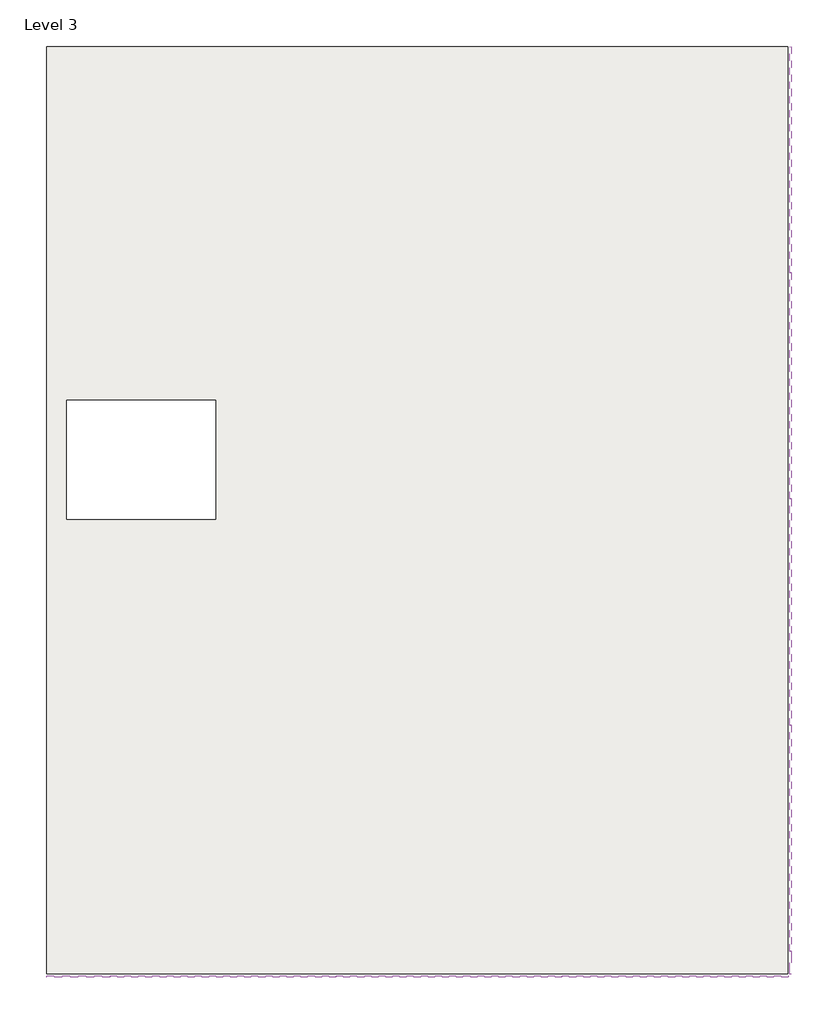
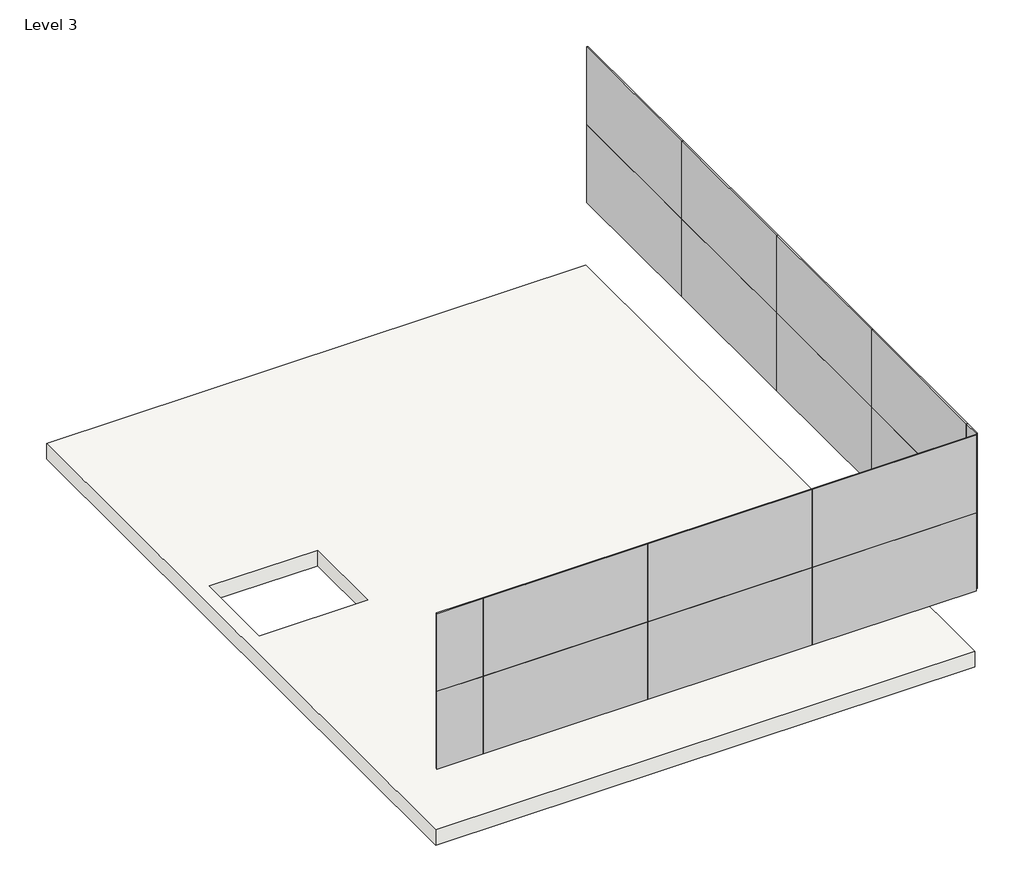
# One storey: 18 plates, 1 slab.
"""IFC4 building model written with IfcOpenShell, lengths in millimetres."""

import ifcopenshell
import ifcopenshell.guid

model = None  # the IFC model being written
_history = None  # IfcOwnerHistory: only IFC2X3 demands one
_inside = {}  # id of a spatial element -> (the spatial element, [elements in it])
_under = {}  # id of a project, library or spatial element -> (it, [spatial elements below it])
_declared = {}  # id of a project -> (the project, [libraries it declares])
_typed = {}  # id of a type object -> (the type object, [elements of that type])
_made_of = {}  # id of a material, layer set ... -> (it, [elements and type objects made of it])


def new_model(schema):
    """Start an empty IFC model of exactly this schema.

    Asked for "IFC4X3", IfcOpenShell would pick the latest addendum, in which some entities
    have other attributes; the version numbers below select the first issue.
    IFC2X3 requires an IfcOwnerHistory on every rooted entity: one is made here for all.
    """
    global model, _history
    if schema == "IFC4X3":
        model = ifcopenshell.file(schema_version=(4, 3, 0, 0))
    else:
        model = ifcopenshell.file(schema=schema)
    _inside.clear()
    _under.clear()
    _declared.clear()
    _typed.clear()
    _made_of.clear()
    _history = None
    if model.schema == "IFC2X3":
        org = make("IfcOrganization", Name="unknown")
        user = make(
            "IfcPersonAndOrganization",
            ThePerson=make("IfcPerson", FamilyName="unknown"),
            TheOrganization=org,
        )
        app = make(
            "IfcApplication",
            ApplicationDeveloper=org,
            Version="unknown",
            ApplicationFullName="unknown",
            ApplicationIdentifier="unknown",
        )
        _history = make(
            "IfcOwnerHistory",
            OwningUser=user,
            OwningApplication=app,
            ChangeAction="ADDED",
            CreationDate=0,
        )
    return model


def make(cls, **values):
    """One entity of the class cls with the attributes given. An attribute that is None is left unset."""
    return model.create_entity(
        cls, **{name: value for name, value in values.items() if value is not None}
    )


def rooted(cls, **values):
    """An entity with a GlobalId (a new one), such as an element, a storey or a relation."""
    return make(cls, GlobalId=ifcopenshell.guid.new(), OwnerHistory=_history, **values)


def si_unit(unit_type, name, prefix=None):
    """IfcSIUnit, for example si_unit("LENGTHUNIT", "METRE", prefix="MILLI")."""
    return make("IfcSIUnit", UnitType=unit_type, Prefix=prefix, Name=name)


def assignment(units):
    """IfcUnitAssignment: the units of a project."""
    return None if units is None else make("IfcUnitAssignment", Units=units)


def point(xyz):
    """IfcCartesianPoint."""
    return None if xyz is None else make("IfcCartesianPoint", Coordinates=xyz)


def direction(xyz):
    """IfcDirection."""
    return None if xyz is None else make("IfcDirection", DirectionRatios=xyz)


def frame(location, z_axis=None, x_axis=None):
    """IfcAxis2Placement3D, a coordinate frame: its origin and axes. An axis left out is left unset."""
    return make(
        "IfcAxis2Placement3D",
        Location=point(location),
        Axis=direction(z_axis),
        RefDirection=direction(x_axis),
    )


def origin():
    """The frame at (0, 0, 0) with its axes left unset."""
    return frame((0.0, 0.0, 0.0))


def origin_with_axes():
    """The frame at (0, 0, 0) with the z axis (0, 0, 1) and the x axis (1, 0, 0) written out."""
    return frame((0.0, 0.0, 0.0), z_axis=(0.0, 0.0, 1.0), x_axis=(1.0, 0.0, 0.0))


def place(relative_to, where):
    """IfcLocalPlacement: puts the frame where relative to a parent placement (None: the world)."""
    return make(
        "IfcLocalPlacement", PlacementRelTo=relative_to, RelativePlacement=where
    )


def context(
    kind, dimensions, precision=None, world=None, true_north=None, identifier=None
):
    """IfcGeometricRepresentationContext, for example the 3D "Model" context."""
    return make(
        "IfcGeometricRepresentationContext",
        ContextIdentifier=identifier,
        ContextType=kind,
        CoordinateSpaceDimension=dimensions,
        Precision=precision,
        WorldCoordinateSystem=world,
        TrueNorth=true_north,
    )


def project(units=None, contexts=None):
    """IfcProject with its units and contexts."""
    return rooted(
        "IfcProject",
        Name="project",
        RepresentationContexts=contexts,
        UnitsInContext=assignment(units),
    )


def spatial(cls, under=None, at=None, **own):
    """A site, building, storey or space (cls), placed at a placement, below another one or the project."""
    s = rooted(cls, ObjectPlacement=at, **own)
    if under is not None:
        _under.setdefault(under.id(), (under, []))[1].append(s)
    return s


def polyline(points):
    """IfcPolyline through the points."""
    return make("IfcPolyline", Points=[point(p) for p in points])


def outline(outer, holes=None, kind="AREA"):
    """IfcArbitraryClosedProfileDef: a profile drawn as a closed curve; with holes, ...WithVoids."""
    if holes is None:
        return make("IfcArbitraryClosedProfileDef", ProfileType=kind, OuterCurve=outer)
    return make(
        "IfcArbitraryProfileDefWithVoids",
        ProfileType=kind,
        OuterCurve=outer,
        InnerCurves=holes,
    )


def extrude(swept, where, along, depth):
    """IfcExtrudedAreaSolid: the profile swept, set in the frame where, extruded along a direction by depth."""
    return make(
        "IfcExtrudedAreaSolid",
        SweptArea=swept,
        Position=where,
        ExtrudedDirection=direction(along),
        Depth=depth,
    )


def shape(context_of_items, identifier, shape_type, items):
    """IfcShapeRepresentation: the items that make up one representation, for example the "Body"."""
    return make(
        "IfcShapeRepresentation",
        ContextOfItems=context_of_items,
        RepresentationIdentifier=identifier,
        RepresentationType=shape_type,
        Items=items,
    )


def source(mapping_origin, context_of_items, identifier, shape_type, items):
    """IfcRepresentationMap: a shape defined once, which mapped items show again and again."""
    return make(
        "IfcRepresentationMap",
        MappingOrigin=mapping_origin,
        MappedRepresentation=shape(context_of_items, identifier, shape_type, items),
    )


def transform(
    local_origin,
    x_axis=None,
    y_axis=None,
    z_axis=None,
    scale=None,
    scale2=None,
    scale3=None,
    uniform=True,
):
    """IfcCartesianTransformationOperator3D, or its non-uniform kind. x_axis, y_axis, z_axis: its Axis1, 2, 3."""
    if uniform:
        return make(
            "IfcCartesianTransformationOperator3D",
            Axis1=direction(x_axis),
            Axis2=direction(y_axis),
            LocalOrigin=point(local_origin),
            Scale=scale,
            Axis3=direction(z_axis),
        )
    return make(
        "IfcCartesianTransformationOperator3DnonUniform",
        Axis1=direction(x_axis),
        Axis2=direction(y_axis),
        LocalOrigin=point(local_origin),
        Scale=scale,
        Axis3=direction(z_axis),
        Scale2=scale2,
        Scale3=scale3,
    )


def mapped(mapping_source, mapping_target):
    """IfcMappedItem: shows the shape of a source again, moved by a transform."""
    return make(
        "IfcMappedItem", MappingSource=mapping_source, MappingTarget=mapping_target
    )


def made_of(thing, what):
    """Note that an element or type object is made of a material, layer set ...; save() writes the relation."""
    if what is not None:
        _made_of.setdefault(what.id(), (what, []))[1].append(thing)
    return thing


def element(
    cls,
    number,
    at=None,
    inside=None,
    cuts=None,
    type_object=None,
    material=None,
    context=None,
    identifier="Body",
    shape_type=None,
    held_by="IfcProductDefinitionShape",
    body=None,
    shapes=None,
    **own,
):
    """One element of the class cls, such as IfcWall. Its Tag is "e" and its number.

    at: its placement. inside: the storey or other place that contains it. cuts: it is an
    opening in that element (IfcRelVoidsElement). A single representation is given by context,
    identifier, shape_type and body (its items); several are given by shapes. held_by: the class
    of the entity that holds the representations. save() writes the other relations.
    """
    e = rooted(cls, Tag="e%d" % number, ObjectPlacement=at, **own)
    if body is not None:
        shapes = [shape(context, identifier, shape_type, body)]
    if shapes is not None:
        e.Representation = make(held_by, Representations=shapes)
    if inside is not None:
        _inside.setdefault(inside.id(), (inside, []))[1].append(e)
    if cuts is not None:
        rooted(
            "IfcRelVoidsElement", RelatingBuildingElement=cuts, RelatedOpeningElement=e
        )
    if type_object is not None:
        _typed.setdefault(type_object.id(), (type_object, []))[1].append(e)
    return made_of(e, material)


def aggregate(whole, parts):
    """IfcRelAggregates: a whole, such as a stair, and the parts it consists of."""
    return rooted("IfcRelAggregates", RelatingObject=whole, RelatedObjects=parts)


def save(model, path):
    """Write the relations noted so far, then the file.

    IfcRelAggregates (storeys below a building ...), IfcRelContainedInSpatialStructure (elements
    in a storey), IfcRelDefinesByType, IfcRelAssociatesMaterial and IfcRelDeclares: one each for
    every whole, place, type object, material and project.
    """
    for whole, parts in _under.values():
        aggregate(whole, parts)
    for where, things in _inside.values():
        rooted(
            "IfcRelContainedInSpatialStructure",
            RelatedElements=things,
            RelatingStructure=where,
        )
    for kind, things in _typed.values():
        rooted("IfcRelDefinesByType", RelatedObjects=things, RelatingType=kind)
    for what, things in _made_of.values():
        rooted("IfcRelAssociatesMaterial", RelatedObjects=things, RelatingMaterial=what)
    for by, libraries in _declared.values():
        rooted("IfcRelDeclares", RelatingContext=by, RelatedDefinitions=libraries)
    model.write(path)


def system_panel_glazed_1e57f9bb(model_context):
    return source(origin(), model_context, "Body", "SweptSolid", [
        extrude(outline(polyline([(1524.0000002, 19.05), (-1524.0000002, 19.05), (-1524.0000002, 44.45), (1524.0000002, 44.45), (1524.0000002, 19.05)])), origin_with_axes(), (0.0, 0.0, 1.0), 1524.0),
    ])


def system_panel_glazed_ccfd9adb(model_context):
    return source(origin(), model_context, "Body", "SweptSolid", [
        extrude(outline(polyline([(427.9999998, 19.05), (-427.9999998, 19.05), (-427.9999998, 44.45), (427.9999998, 44.45), (427.9999998, 19.05)])), origin_with_axes(), (0.0, 0.0, 1.0), 1524.0),
    ])


def system_panel_glazed_88f24eba(model_context):
    return source(origin(), model_context, "Body", "SweptSolid", [
        extrude(outline(polyline([(153.9999998, 19.05), (-153.9999998, 19.05), (-153.9999998, 44.45), (153.9999998, 44.45), (153.9999998, 19.05)])), origin_with_axes(), (0.0, 0.0, 1.0), 1524.0),
    ])


model = new_model("IFC4")

# Units and contexts
model_context = context("Model", 3, world=origin())
ifc_project = project(units=[si_unit("LENGTHUNIT", "METRE", prefix="MILLI")], contexts=[model_context])

# Site, building, storey
site = spatial("IfcSite", under=ifc_project)
building = spatial("IfcBuilding", under=site)
storey = spatial("IfcBuildingStorey", under=building, Name="Level 3", Elevation=6400.0)

# Plates
placement = place(None, origin())
system_panel_glazed_shape = system_panel_glazed_1e57f9bb(model_context)
element("IfcPlate", 1, ObjectType="System Panel : Glazed", at=placement, inside=storey, context=model_context, shape_type="MappedRepresentation", body=[
    mapped(system_panel_glazed_shape, transform((2137.6340362, 1399.6955828, 7620.0), x_axis=(-1.0, 0.0, 0.0), y_axis=(0.0, -1.0, 0.0), z_axis=(0.0, 0.0, 1.0))),
])
element("IfcPlate", 2, ObjectType="System Panel : Glazed", at=placement, inside=storey, context=model_context, shape_type="MappedRepresentation", body=[
    mapped(system_panel_glazed_shape, transform((-910.3659639, 1399.6955828, 7620.0), x_axis=(-1.0, 0.0, 0.0), y_axis=(0.0, -1.0, 0.0), z_axis=(0.0, 0.0, 1.0))),
])
element("IfcPlate", 3, ObjectType="System Panel : Glazed", at=placement, inside=storey, context=model_context, shape_type="MappedRepresentation", body=[
    mapped(system_panel_glazed_shape, transform((-3958.3659639, 1399.6955828, 7620.0), x_axis=(-1.0, 0.0, 0.0), y_axis=(0.0, -1.0, 0.0), z_axis=(0.0, 0.0, 1.0))),
])
element("IfcPlate", 4, ObjectType="System Panel : Glazed", at=placement, inside=storey, context=model_context, shape_type="MappedRepresentation", body=[
    mapped(system_panel_glazed_shape, transform((2137.6340362, 1399.6955828, 9144.0), x_axis=(-1.0, 0.0, 0.0), y_axis=(0.0, -1.0, 0.0), z_axis=(0.0, 0.0, 1.0))),
])
element("IfcPlate", 5, ObjectType="System Panel : Glazed", at=placement, inside=storey, context=model_context, shape_type="MappedRepresentation", body=[
    mapped(system_panel_glazed_shape, transform((-910.3659639, 1399.6955828, 9144.0), x_axis=(-1.0, 0.0, 0.0), y_axis=(0.0, -1.0, 0.0), z_axis=(0.0, 0.0, 1.0))),
])
element("IfcPlate", 6, ObjectType="System Panel : Glazed", at=placement, inside=storey, context=model_context, shape_type="MappedRepresentation", body=[
    mapped(system_panel_glazed_shape, transform((-3958.3659639, 1399.6955828, 9144.0), x_axis=(-1.0, 0.0, 0.0), y_axis=(0.0, -1.0, 0.0), z_axis=(0.0, 0.0, 1.0))),
])
element("IfcPlate", 7, ObjectType="System Panel : Glazed", at=placement, inside=storey, context=model_context, shape_type="MappedRepresentation", body=[
    mapped(system_panel_glazed_shape, transform((3661.6340364, 12375.6955827, 7620.0), x_axis=(0.0, -1.0, 0.0), y_axis=(1.0, 0.0, 0.0), z_axis=(0.0, 0.0, 1.0))),
])
element("IfcPlate", 8, ObjectType="System Panel : Glazed", at=placement, inside=storey, context=model_context, shape_type="MappedRepresentation", body=[
    mapped(system_panel_glazed_shape, transform((3661.6340364, 9327.6955825, 7620.0), x_axis=(0.0, -1.0, 0.0), y_axis=(1.0, 0.0, 0.0), z_axis=(0.0, 0.0, 1.0))),
])
element("IfcPlate", 9, ObjectType="System Panel : Glazed", at=placement, inside=storey, context=model_context, shape_type="MappedRepresentation", body=[
    mapped(system_panel_glazed_shape, transform((3661.6340364, 6279.6955825, 7620.0), x_axis=(0.0, -1.0, 0.0), y_axis=(1.0, 0.0, 0.0), z_axis=(0.0, 0.0, 1.0))),
])
element("IfcPlate", 10, ObjectType="System Panel : Glazed", at=placement, inside=storey, context=model_context, shape_type="MappedRepresentation", body=[
    mapped(system_panel_glazed_shape, transform((3661.6340364, 3231.6955825, 7620.0), x_axis=(0.0, -1.0, 0.0), y_axis=(1.0, 0.0, 0.0), z_axis=(0.0, 0.0, 1.0))),
])
element("IfcPlate", 11, ObjectType="System Panel : Glazed", at=placement, inside=storey, context=model_context, shape_type="MappedRepresentation", body=[
    mapped(system_panel_glazed_shape, transform((3661.6340364, 12375.6955827, 9144.0), x_axis=(0.0, -1.0, 0.0), y_axis=(1.0, 0.0, 0.0), z_axis=(0.0, 0.0, 1.0))),
])
element("IfcPlate", 12, ObjectType="System Panel : Glazed", at=placement, inside=storey, context=model_context, shape_type="MappedRepresentation", body=[
    mapped(system_panel_glazed_shape, transform((3661.6340364, 9327.6955825, 9144.0), x_axis=(0.0, -1.0, 0.0), y_axis=(1.0, 0.0, 0.0), z_axis=(0.0, 0.0, 1.0))),
])
element("IfcPlate", 13, ObjectType="System Panel : Glazed", at=placement, inside=storey, context=model_context, shape_type="MappedRepresentation", body=[
    mapped(system_panel_glazed_shape, transform((3661.6340364, 6279.6955825, 9144.0), x_axis=(0.0, -1.0, 0.0), y_axis=(1.0, 0.0, 0.0), z_axis=(0.0, 0.0, 1.0))),
])
element("IfcPlate", 14, ObjectType="System Panel : Glazed", at=placement, inside=storey, context=model_context, shape_type="MappedRepresentation", body=[
    mapped(system_panel_glazed_shape, transform((3661.6340364, 3231.6955825, 9144.0), x_axis=(0.0, -1.0, 0.0), y_axis=(1.0, 0.0, 0.0), z_axis=(0.0, 0.0, 1.0))),
])
system_panel_glazed_2_shape = system_panel_glazed_ccfd9adb(model_context)
element("IfcPlate", 15, ObjectType="System Panel : Glazed", at=placement, inside=storey, context=model_context, shape_type="MappedRepresentation", body=[
    mapped(system_panel_glazed_2_shape, transform((-5910.3659638, 1399.6955828, 7620.0), x_axis=(-1.0, 0.0, 0.0), y_axis=(0.0, -1.0, 0.0), z_axis=(0.0, 0.0, 1.0))),
])
element("IfcPlate", 16, ObjectType="System Panel : Glazed", at=placement, inside=storey, context=model_context, shape_type="MappedRepresentation", body=[
    mapped(system_panel_glazed_2_shape, transform((-5910.3659638, 1399.6955828, 9144.0), x_axis=(-1.0, 0.0, 0.0), y_axis=(0.0, -1.0, 0.0), z_axis=(0.0, 0.0, 1.0))),
])
system_panel_glazed_3_shape = system_panel_glazed_88f24eba(model_context)
element("IfcPlate", 17, ObjectType="System Panel : Glazed", at=placement, inside=storey, context=model_context, shape_type="MappedRepresentation", body=[
    mapped(system_panel_glazed_3_shape, transform((3661.6340364, 1553.6955827, 7620.0), x_axis=(0.0, -1.0, 0.0), y_axis=(1.0, 0.0, 0.0), z_axis=(0.0, 0.0, 1.0))),
])
element("IfcPlate", 18, ObjectType="System Panel : Glazed", at=placement, inside=storey, context=model_context, shape_type="MappedRepresentation", body=[
    mapped(system_panel_glazed_3_shape, transform((3661.6340364, 1553.6955827, 9144.0), x_axis=(0.0, -1.0, 0.0), y_axis=(1.0, 0.0, 0.0), z_axis=(0.0, 0.0, 1.0))),
])

# Slab
element("IfcSlab", 19, ObjectType="Generic - 12\"", at=placement, inside=storey, context=model_context, shape_type="SweptSolid", body=[
    extrude(outline(polyline([(-6335.3659636, 1402.6955828), (-6335.3659636, 13896.6955828), (3658.6340364, 13896.6955828), (3658.6340364, 1402.6955828), (-6335.3659636, 1402.6955828)]), holes=[polyline([(-4059.8993101, 7527.9023719), (-4059.8993101, 9133.9023719), (-6065.8993101, 9133.9023719), (-6065.8993101, 7527.9023719), (-4059.8993101, 7527.9023719)])]), frame((0.0, 0.0, 6095.2), z_axis=(0.0, 0.0, 1.0), x_axis=(1.0, 0.0, 0.0)), (0.0, 0.0, 1.0), 304.8),
])

save(model, "model.ifc")

# Revit data of these elements
# Type "System Panel : Glazed"
#   Construction Type Id = "GSP4R"
#   Analytic Construction = "1/8 in Pilkington single glazing"
#   Visual Light Transmittance = 0.9
#   Solar Heat Gain Coefficient = 0.86
#   Heat Transfer Coefficient (U) = 6.7069 W/(m²·K)
# Type "Generic - 12\""
#   Assembly Code = "B1010"
#   Function = 0
#   Layers, outside or top first: 0.3048 m no material (function 1)
# Elements 1, 2, 3, 4, 5, 6, 7, 8, 9, 10, 11, 12, 13, 14, 15, 16, 17, 18 (IfcPlate, "System Panel : Glazed")
#   Phase Created = New Construction
#   Materials on its faces: "Glass"
# Element 19 (IfcSlab, "Generic - 12\"")
#   built-in parameter 1001955 = -1.5708 (stored number, unit not read)
#   Height Offset From Level = 0.00 m
#   Phase Created = New Construction
#   Materials on its faces: "Default Floor"
# Materials
#   "Glass": class "Glass", colour RGB 0 128 192, transparency 0.75, Description = "Soda Lime Glass", Cost = 0
#   "Default Floor": class "Miscellaneous", colour RGB 128 128 128, transparency 0, Cost = 0
